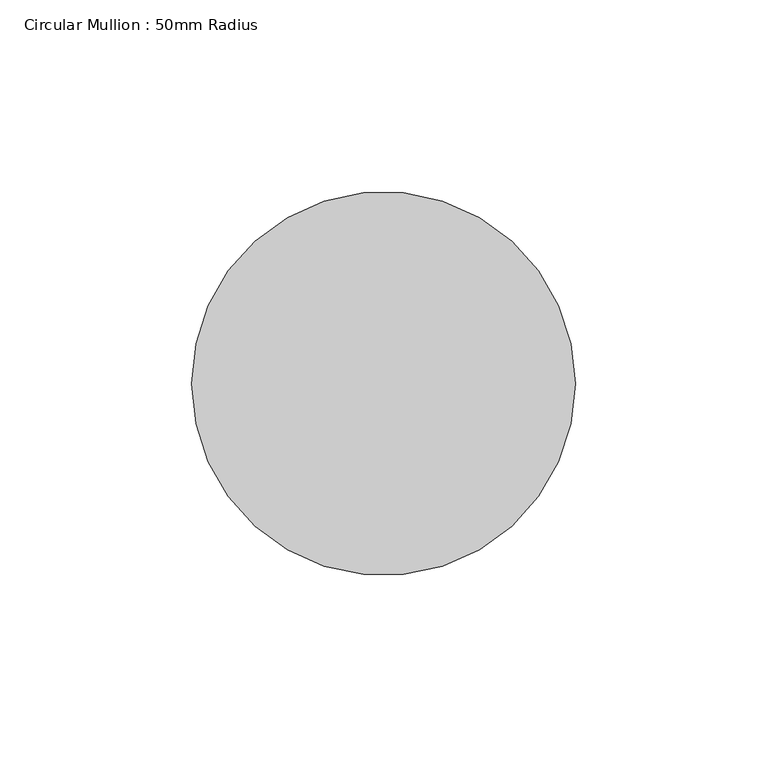
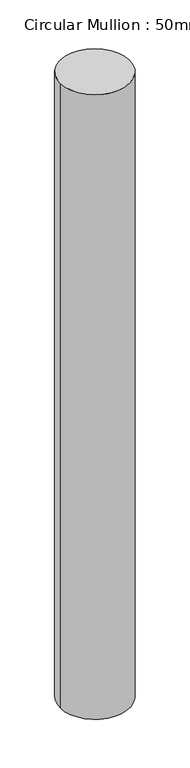
"""IFC4 building model written with IfcOpenShell, lengths in millimetres: member geometry, Circular Mullion : 50mm Radius."""

from ifc_helpers import new_model, si_unit, point, frame, origin, origin_2d, place, context, project, spatial, circle_curve, trimmed, segment, composite_curve, outline, extrude, source, transform, mapped, element, save


def circular_mullion_50mm_radius_7b24aeea(model_context):
    return source(origin(), model_context, "Body", "SweptSolid", [
        extrude(outline(composite_curve([segment(trimmed(circle_curve(origin_2d(), 50.0), [point((50.0, 0.0))], [point((-50.0, 0.0))], False, "CARTESIAN"), True, "CONTINUOUS"), segment(trimmed(circle_curve(origin_2d(), 50.0), [point((-50.0, 0.0))], [point((50.0, 0.0))], False, "CARTESIAN"), True, "CONTINUOUS")], self_intersect=False)), frame((0.0, 0.0, -948.6163978), z_axis=(0.0, 0.0, 1.0), x_axis=(1.0, 0.0, 0.0)), (0.0, 0.0, 1.0), 948.6163978),
    ])


if __name__ == "__main__":
    model = new_model("IFC4")
    model_context = context("Model", 3, world=origin())
    ifc_project = project(units=[si_unit("LENGTHUNIT", "METRE", prefix="MILLI")], contexts=[model_context])
    site = spatial("IfcSite", under=ifc_project)
    building = spatial("IfcBuilding", under=site)
    placement = place(None, origin())
    circular_mullion_50mm_radius_shape = circular_mullion_50mm_radius_7b24aeea(model_context)
    element("IfcMember", 1, ObjectType="Circular Mullion : 50mm Radius", at=placement, inside=building, context=model_context, shape_type="MappedRepresentation", body=[
        mapped(circular_mullion_50mm_radius_shape, transform((0.0, 0.0, 0.0), x_axis=(1.0, 0.0, 0.0), y_axis=(0.0, 1.0, 0.0), z_axis=(0.0, 0.0, 1.0))),
    ])
    save(model, "model.ifc")

# Revit data of these elements
# Type "Circular Mullion : 50mm Radius"
#   built-in parameter 1007350 = 0.164042 (stored number, unit not read)
# Element 1 (IfcMember, "Circular Mullion : 50mm Radius")
#   Materials on its faces: "Aluminium"
# Materials
#   "Aluminium": class "Metal", colour RGB 247 247 247, transparency 0, Description = "Aluminium 6061", Cost = 0
